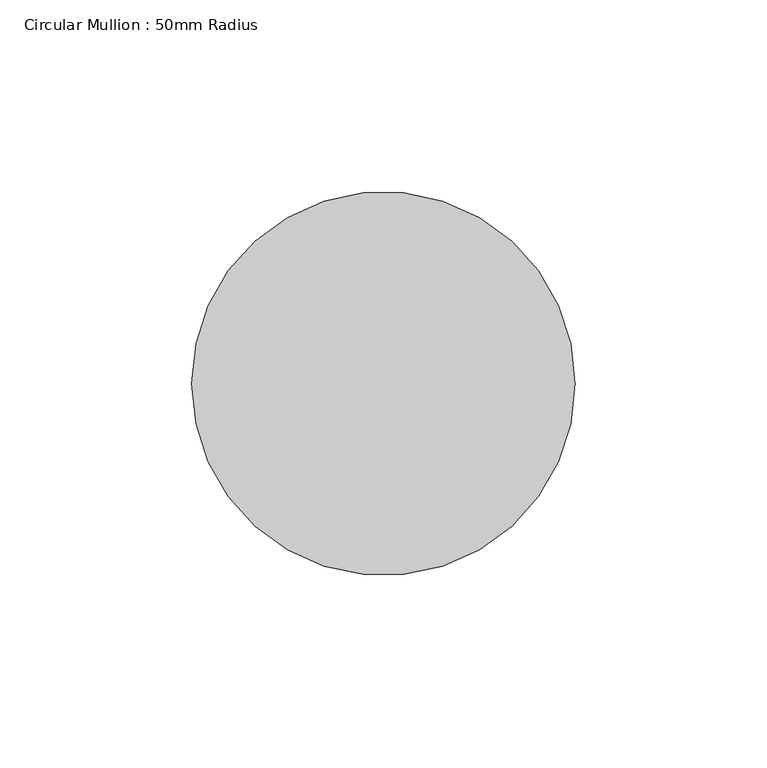
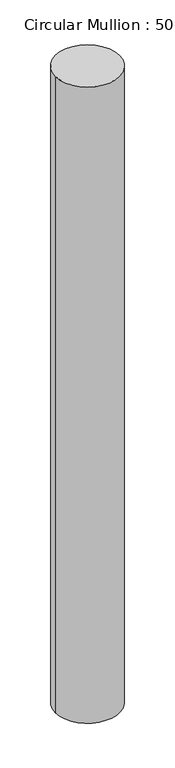
"""IFC4 building model written with IfcOpenShell, lengths in millimetres: member geometry, Circular Mullion : 50mm Radius."""

from ifc_helpers import new_model, si_unit, point, frame, origin, origin_2d, place, context, project, spatial, circle_curve, trimmed, segment, composite_curve, outline, extrude, source, transform, mapped, element, save


def circular_mullion_50mm_radius_ff95a933(model_context):
    return source(origin(), model_context, "Body", "SweptSolid", [
        extrude(outline(composite_curve([segment(trimmed(circle_curve(origin_2d(), 50.0), [point((50.0, 0.0))], [point((-50.0, 0.0))], False, "CARTESIAN"), True, "CONTINUOUS"), segment(trimmed(circle_curve(origin_2d(), 50.0), [point((-50.0, 0.0))], [point((50.0, 0.0))], False, "CARTESIAN"), True, "CONTINUOUS")], self_intersect=False)), frame((0.0, 0.0, -1051.0728006), z_axis=(0.0, 0.0, 1.0), x_axis=(1.0, 0.0, 0.0)), (0.0, 0.0, 1.0), 1051.0728006),
    ])


if __name__ == "__main__":
    model = new_model("IFC4")
    model_context = context("Model", 3, world=origin())
    ifc_project = project(units=[si_unit("LENGTHUNIT", "METRE", prefix="MILLI")], contexts=[model_context])
    site = spatial("IfcSite", under=ifc_project)
    building = spatial("IfcBuilding", under=site)
    placement = place(None, origin())
    circular_mullion_50mm_radius_shape = circular_mullion_50mm_radius_ff95a933(model_context)
    element("IfcMember", 1, ObjectType="Circular Mullion : 50mm Radius", at=placement, inside=building, context=model_context, shape_type="MappedRepresentation", body=[
        mapped(circular_mullion_50mm_radius_shape, transform((0.0, 0.0, 0.0), x_axis=(1.0, 0.0, 0.0), y_axis=(0.0, 1.0, 0.0), z_axis=(0.0, 0.0, 1.0))),
    ])
    save(model, "model.ifc")

# Revit data of these elements
# Type "Circular Mullion : 50mm Radius"
#   built-in parameter 1007350 = 0.164042 (stored number, unit not read)
# Element 1 (IfcMember, "Circular Mullion : 50mm Radius")
#   Materials on its faces: "Aluminium"
# Materials
#   "Aluminium": class "Metal", colour RGB 247 247 247, transparency 0, Description = "Aluminium 6061", Cost = 0
